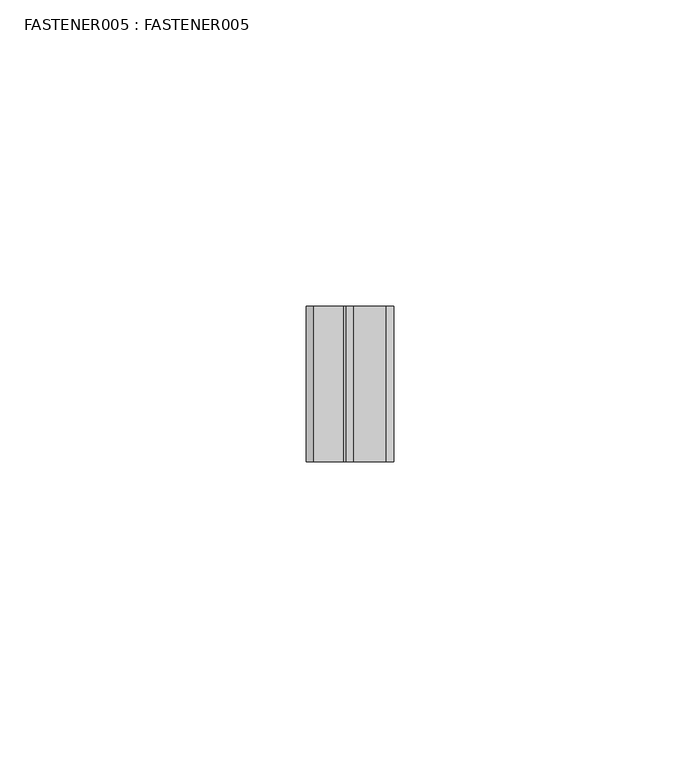
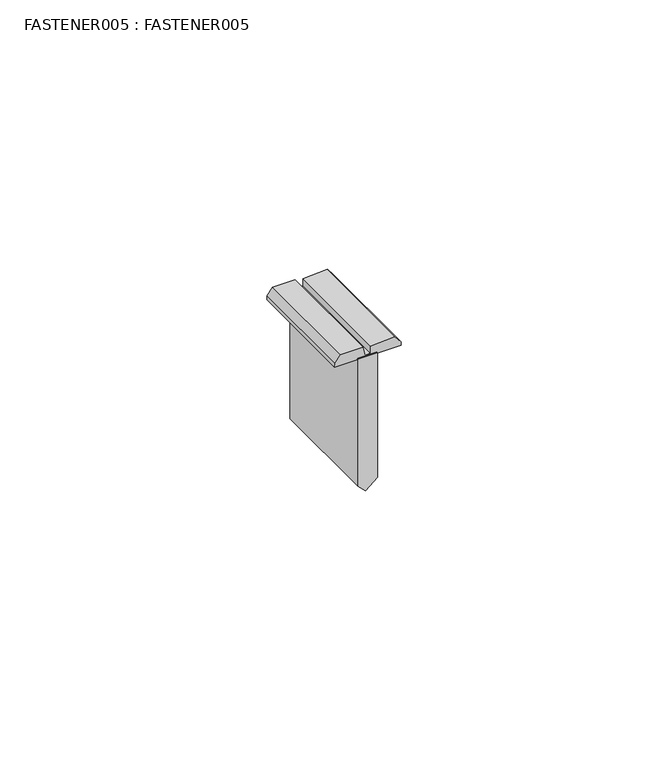
"""IFC4 building model written with IfcOpenShell, lengths in millimetres: proxy geometry, FASTENER005 : FASTENER005."""

from ifc_helpers import new_model, si_unit, frame, origin, place, context, project, spatial, polyline, outline, extrude, source, transform, mapped, element, save


def fastener005_fastener005_4a0cef2c(model_context):
    return source(origin(), model_context, "Body", "SweptSolid", [
        extrude(outline(polyline([(42579.6987049, 5977.3107075), (42550.7399648, 5977.3107075), (42549.1244121, 5978.9677221), (42551.3049701, 5981.517626), (42579.6987049, 5981.517626), (42579.6987049, 5977.3107075)])), frame((0.0, -1078.2906574, 0.0), z_axis=(0.0, 1.0, 0.0), x_axis=(0.0, 0.0, 1.0)), (0.0, 0.0, 1.0), 25.4),
        extrude(outline(polyline([(42579.6987049, 5986.5634932), (42580.508527, 5986.5634932), (42582.1023984, 5985.3247911), (42581.7061629, 5980.0391089), (42580.1167322, 5980.0391089), (42580.1167322, 5978.792004), (42582.1288635, 5978.3957685), (42582.1288635, 5973.5166866), (42580.5349921, 5972.2779845), (42579.6987049, 5972.2671879), (42579.6987049, 5986.5634932)])), frame((0.0, -1078.2906574, 0.0), z_axis=(0.0, 1.0, 0.0), x_axis=(0.0, 0.0, 1.0)), (0.0, 0.0, 1.0), 25.4),
    ])


if __name__ == "__main__":
    model = new_model("IFC4")
    model_context = context("Model", 3, world=origin())
    ifc_project = project(units=[si_unit("LENGTHUNIT", "METRE", prefix="MILLI")], contexts=[model_context])
    site = spatial("IfcSite", under=ifc_project)
    building = spatial("IfcBuilding", under=site)
    placement = place(None, origin())
    fastener005_fastener005_shape = fastener005_fastener005_4a0cef2c(model_context)
    element("IfcBuildingElementProxy", 1, Name="FASTENER005 : FASTENER005", ObjectType="FASTENER005 : FASTENER005", at=placement, inside=building, context=model_context, shape_type="MappedRepresentation", body=[
        mapped(fastener005_fastener005_shape, transform((0.0, 0.0, 0.0), x_axis=(1.0, 0.0, 0.0), y_axis=(0.0, 1.0, 0.0), z_axis=(0.0, 0.0, 1.0))),
    ])
    save(model, "model.ifc")

# Revit data of these elements
# Type "FASTENER005 : FASTENER005"
#   NameOverride = "FASTENER005"
# Element 1 (IfcBuildingElementProxy, "FASTENER005 : FASTENER005")
#   Materials on its faces: "ENGINEERED PANCAKE HEAD FASTENER @ 12\" O.C."
# Materials
#   "ENGINEERED PANCAKE HEAD FASTENER @ 12\" O.C.": class "Unassigned", colour RGB 255 255 255, transparency 0, Cost = 0
